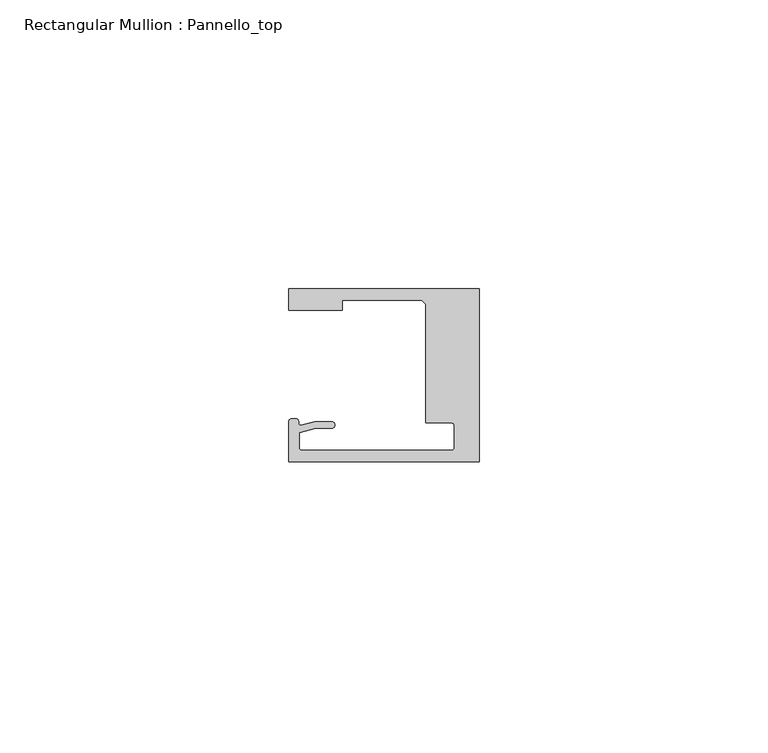
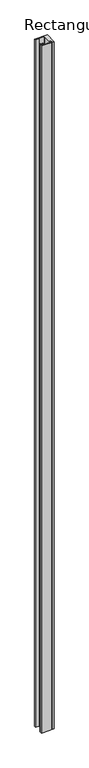
"""IFC4 building model written with IfcOpenShell, lengths in millimetres: member geometry, Rectangular Mullion : Pannello_top."""

from ifc_helpers import new_model, si_unit, frame, origin, place, context, project, spatial, polyline, circle_curve, source, transform, mapped, element, save
from ifc_brep_helpers import plane_surface, cylinder_surface, revolved_surface, extruded_surface, spline_curve, advanced_brep


def rectangular_mullion_pannello_top_d634514d(model_context):
    return source(origin(), model_context, "Body", "AdvancedBrep", [
        advanced_brep(
        [(-33.0, 15.0, 0.0), (-33.0, 11.3000004, 0.0), (-23.700041, 11.3000004, 0.0), (-23.700041, 13.0000004, 0.0), (-10.0000103, 13.0000004, 0.0), (-9.2999726, 12.2999849, 0.0), (-9.2999726, -8.2500595, 0.0), (-4.7999726, -8.2500595, 0.0), (-4.2999726, -8.7500595, 0.0), (-4.2999726, -12.50001, 0.0), (-4.7999726, -13.00001, 0.0), (-30.69998, -13.00001, 0.0), (-31.19998, -12.50001, 0.0), (-31.19998, -9.9657591, 0.0), (-28.3419477, -9.1999523, 0.0), (-25.59998, -9.1999523, 0.0), (-25.59998, -7.9999523, 0.0), (-28.4999305, -7.9999523, 0.0), (-30.9223017, -8.6490241, 0.0), (-33.0000135, -8.0000472, 0.0), (-33.0000135, -15.0, 0.0), (0.0, -15.0, 0.0), (0.0, 15.0, 0.0), (-33.0, 15.0, -1883.9999729), (0.0, 15.0, -1883.9999729), (0.0, -15.0, -1883.9999729), (-33.0000135, -15.0, -1883.9999729), (-33.0000135, -8.0000472, -1883.9999729), (-30.9223017, -8.6490241, -1883.9999729), (-28.4999305, -7.9999523, -1883.9999729), (-25.59998, -7.9999523, -1883.9999729), (-25.59998, -9.1999523, -1883.9999729), (-28.3419477, -9.1999523, -1883.9999729), (-31.19998, -9.9657591, -1883.9999729), (-31.19998, -12.50001, -1883.9999729), (-30.69998, -13.00001, -1883.9999729), (-4.7999726, -13.00001, -1883.9999729), (-4.2999726, -12.50001, -1883.9999729), (-4.2999726, -8.7500595, -1883.9999729), (-4.7999726, -8.2500595, -1883.9999729), (-9.2999726, -8.2500595, -1883.9999729), (-9.2999726, 12.2999849, -1883.9999729), (-10.0000103, 13.0000004, -1883.9999729), (-23.700041, 13.0000004, -1883.9999729), (-23.700041, 11.3000004, -1883.9999729), (-33.0, 11.3000004, -1883.9999729)],
        [
            (0, 1),
            (1, 2),
            (2, 3),
            (3, 4),
            (4, 5),
            (5, 6),
            (6, 7),
            (7, 8, circle_curve(frame((-4.7999726, -8.7500595, 0.0), z_axis=(0.0, 0.0, -1.0), x_axis=(0.0, 1.0, 0.0)), 0.5)),
            (8, 9),
            (9, 10, circle_curve(frame((-4.7999726, -12.50001, 0.0), z_axis=(0.0, 0.0, -1.0), x_axis=(1.0, 0.0, 0.0)), 0.5)),
            (10, 11),
            (11, 12, circle_curve(frame((-30.69998, -12.50001, 0.0), z_axis=(0.0, 0.0, -1.0), x_axis=(0.0, -1.0, 0.0)), 0.5)),
            (12, 13),
            (13, 14),
            (14, 15),
            (15, 16, circle_curve(frame((-25.59998, -8.5999523, 0.0), z_axis=(0.0, 0.0, 1.0), x_axis=(0.0, -1.0, 0.0)), 0.6)),
            (16, 17),
            (17, 18),
            (18, 19, spline_curve(3, [(-30.9223017, -8.6490241, 0.0), (-31.312054066, -8.717747958, 0.0), (-31.298563602, -8.366228555, 0.0), (-31.305645054, -7.690065204, 0.0), (-31.357433266, -7.563996614, 0.0), (-32.262327879, -7.456527435, 0.0), (-33.0000135, -7.457047519, 0.0), (-33.0000135, -8.0000472, 0.0)], [4, 2, 2, 4], [0.0, 0.001840817752199412, 0.004996616814974408, 0.007702013405570312])),
            (19, 20),
            (20, 21),
            (21, 22),
            (22, 0),
            (23, 24),
            (24, 25),
            (25, 26),
            (26, 27),
            (27, 28, spline_curve(3, [(-33.0000135, -8.0000472, -1883.9999729), (-33.0000135, -7.457047519, -1883.9999729), (-32.262327879, -7.456527435, -1883.9999729), (-31.357433266, -7.563996614, -1883.9999729), (-31.305645054, -7.690065204, -1883.9999729), (-31.298563602, -8.366228555, -1883.9999729), (-31.312054066, -8.717747958, -1883.9999729), (-30.9223017, -8.6490241, -1883.9999729)], [4, 2, 2, 4], [0.0, 0.0027053965905959043, 0.0058611956533709, 0.007702013405570312])),
            (28, 29),
            (29, 30),
            (30, 31, circle_curve(frame((-25.59998, -8.5999523, -1883.9999729), z_axis=(0.0, 0.0, -1.0), x_axis=(0.0, -1.0, 0.0)), 0.6)),
            (31, 32),
            (32, 33),
            (33, 34),
            (34, 35, circle_curve(frame((-30.69998, -12.50001, -1883.9999729), z_axis=(0.0, 0.0, 1.0), x_axis=(0.0, -1.0, 0.0)), 0.5)),
            (35, 36),
            (36, 37, circle_curve(frame((-4.7999726, -12.50001, -1883.9999729), z_axis=(0.0, 0.0, 1.0), x_axis=(1.0, 0.0, 0.0)), 0.5)),
            (37, 38),
            (38, 39, circle_curve(frame((-4.7999726, -8.7500595, -1883.9999729), z_axis=(0.0, 0.0, 1.0), x_axis=(0.0, 1.0, 0.0)), 0.5)),
            (39, 40),
            (40, 41),
            (41, 42),
            (42, 43),
            (43, 44),
            (44, 45),
            (45, 23),
            (0, 23),
            (45, 1),
            (44, 2),
            (43, 3),
            (42, 4),
            (41, 5),
            (40, 6),
            (39, 7),
            (38, 8),
            (37, 9),
            (36, 10),
            (35, 11),
            (34, 12),
            (33, 13),
            (32, 14),
            (31, 15),
            (30, 16),
            (29, 17),
            (28, 18),
            (27, 19),
            (26, 20),
            (25, 21),
            (24, 22),
        ],
        [
            plane_surface(frame((0.0, -36.2491502, 0.0), z_axis=(0.0, 0.0, 1.0), x_axis=(-1.0, 0.0, 0.0))),
            plane_surface(frame((0.0, -36.2491502, -1883.9999729), z_axis=(0.0, 0.0, -1.0), x_axis=(-1.0, 0.0, 0.0))),
            plane_surface(frame((-33.0, 15.0, 0.0), z_axis=(-1.0, 0.0, 0.0), x_axis=(0.0, 0.0, -1.0))),
            plane_surface(frame((-33.0, 11.3000004, 0.0), z_axis=(0.0, -1.0, 0.0), x_axis=(0.0, 0.0, -1.0))),
            plane_surface(frame((-23.700041, 11.3000004, 0.0), z_axis=(1.0, 0.0, 0.0), x_axis=(0.0, 0.0, -1.0))),
            plane_surface(frame((-23.700041, 13.0000004, 0.0), z_axis=(0.0, -1.0, 0.0), x_axis=(0.0, 0.0, -1.0))),
            plane_surface(frame((-10.0000103, 13.0000004, 0.0), z_axis=(-0.7070955486277984, -0.7071180135668678, 0.0), x_axis=(0.0, 0.0, -1.0))),
            plane_surface(frame((-9.2999726, 12.2999849, 0.0), z_axis=(-1.0, 0.0, 0.0), x_axis=(0.0, 0.0, -1.0))),
            plane_surface(frame((-9.2999726, -8.2500595, 0.0), z_axis=(0.0, -1.0, 0.0), x_axis=(0.0, 0.0, -1.0))),
            revolved_surface(polyline([(-4.7999726, -8.2500595, -1883.9999729), (-4.7999726, -8.2500595, 0.0)]), (-4.7999726, -8.7500595, 0.0), (0.0, 0.0, -1.0)),
            plane_surface(frame((-4.2999726, -8.7500595, 0.0), z_axis=(-1.0, 0.0, 0.0), x_axis=(0.0, 0.0, -1.0))),
            revolved_surface(polyline([(-4.2999726, -12.50001, -1883.9999729), (-4.2999726, -12.50001, 0.0)]), (-4.7999726, -12.50001, 0.0), (0.0, 0.0, -1.0)),
            plane_surface(frame((-4.7999726, -13.00001, 0.0), z_axis=(0.0, 1.0, 0.0), x_axis=(0.0, 0.0, -1.0))),
            revolved_surface(polyline([(-30.69998, -13.00001, -1883.9999729), (-30.69998, -13.00001, 0.0)]), (-30.69998, -12.50001, 0.0), (0.0, 0.0, -1.0)),
            plane_surface(frame((-31.19998, -12.50001, 0.0), z_axis=(1.0, 0.0, 0.0), x_axis=(0.0, 0.0, -1.0))),
            plane_surface(frame((-31.19998, -9.9657591, 0.0), z_axis=(0.25881883204288636, -0.9659258833782002, 0.0), x_axis=(0.0, 0.0, -1.0))),
            plane_surface(frame((-28.3419477, -9.1999523, 0.0), z_axis=(0.0, -1.0, 0.0), x_axis=(0.0, 0.0, -1.0))),
            cylinder_surface(frame((-25.59998, -8.5999523, 0.0), z_axis=(0.0, 0.0, 1.0), x_axis=(0.0, -1.0, 0.0)), 0.6),
            plane_surface(frame((-25.59998, -7.9999523, 0.0), z_axis=(0.0, 1.0, 0.0), x_axis=(0.0, 0.0, -1.0))),
            plane_surface(frame((-28.4999305, -7.9999523, 0.0), z_axis=(-0.25881883200192934, 0.9659258833891746, 0.0), x_axis=(0.0, 0.0, -1.0))),
            extruded_surface(spline_curve(3, [(-30.9223017, -8.6490241, -1883.9999729), (-31.312054066, -8.717747958, -1883.9999729), (-31.298563602, -8.366228555, -1883.9999729), (-31.305645054, -7.690065204, -1883.9999729), (-31.357433266, -7.563996614, -1883.9999729), (-32.262327879, -7.456527435, -1883.9999729), (-33.0000135, -7.457047519, -1883.9999729), (-33.0000135, -8.0000472, -1883.9999729)], [4, 2, 2, 4], [0.0, 0.001840817752199412, 0.004996616814974408, 0.007702013405570312]), (0.0, 0.0, 1883.9999729), 1883.9999729),
            plane_surface(frame((-33.0000135, -8.0000472, 0.0), z_axis=(-1.0, 0.0, 0.0), x_axis=(0.0, 0.0, -1.0))),
            plane_surface(frame((-33.0000135, -15.0, 0.0), z_axis=(0.0, -1.0, 0.0), x_axis=(0.0, 0.0, -1.0))),
            plane_surface(frame((0.0, -15.0, 0.0), z_axis=(1.0, 0.0, 0.0), x_axis=(0.0, 0.0, -1.0))),
            plane_surface(frame((0.0, 15.0, 0.0), z_axis=(0.0, 1.0, 0.0), x_axis=(0.0, 0.0, -1.0))),
        ],
        [
            (0, [[1, 2, 3, 4, 5, 6, 7, 8, 9, 10, 11, 12, 13, 14, 15, 16, 17, 18, 19, 20, 21, 22, 23]]),
            (1, [[24, 25, 26, 27, 28, 29, 30, 31, 32, 33, 34, 35, 36, 37, 38, 39, 40, 41, 42, 43, 44, 45, 46]]),
            (2, [[-1, 47, -46, 48]]),
            (3, [[-2, -48, -45, 49]]),
            (4, [[-3, -49, -44, 50]]),
            (5, [[-4, -50, -43, 51]]),
            (6, [[-5, -51, -42, 52]]),
            (7, [[-6, -52, -41, 53]]),
            (8, [[-7, -53, -40, 54]]),
            (9, [[-8, -54, -39, 55]]),
            (10, [[-9, -55, -38, 56]]),
            (11, [[-10, -56, -37, 57]]),
            (12, [[-11, -57, -36, 58]]),
            (13, [[-12, -58, -35, 59]]),
            (14, [[-13, -59, -34, 60]]),
            (15, [[-14, -60, -33, 61]]),
            (16, [[-15, -61, -32, 62]]),
            (17, [[-16, -62, -31, 63]]),
            (18, [[-17, -63, -30, 64]]),
            (19, [[-18, -64, -29, 65]]),
            (20, [[-19, -65, -28, 66]]),
            (21, [[-20, -66, -27, 67]]),
            (22, [[-21, -67, -26, 68]]),
            (23, [[-22, -68, -25, 69]]),
            (24, [[-23, -69, -24, -47]]),
        ],
    ),
    ])


if __name__ == "__main__":
    model = new_model("IFC4")
    model_context = context("Model", 3, world=origin())
    ifc_project = project(units=[si_unit("LENGTHUNIT", "METRE", prefix="MILLI")], contexts=[model_context])
    site = spatial("IfcSite", under=ifc_project)
    building = spatial("IfcBuilding", under=site)
    placement = place(None, origin())
    rectangular_mullion_pannello_top_shape = rectangular_mullion_pannello_top_d634514d(model_context)
    element("IfcMember", 1, ObjectType="Rectangular Mullion : Pannello_top", at=placement, inside=building, context=model_context, shape_type="MappedRepresentation", body=[
        mapped(rectangular_mullion_pannello_top_shape, transform((0.0, 0.0, 0.0), x_axis=(1.0, 0.0, 0.0), y_axis=(0.0, 1.0, 0.0), z_axis=(0.0, 0.0, 1.0))),
    ])
    save(model, "model.ifc")

# Revit data of these elements
# Type "Rectangular Mullion : Pannello_top"
#   built-in parameter 1007322 = 0.0984252 (stored number, unit not read)
#   built-in parameter 1007321 = 0 (stored number, unit not read)
#   built-in parameter 1007320 = 0.0305117 (stored number, unit not read)
